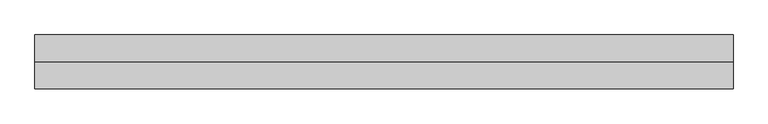
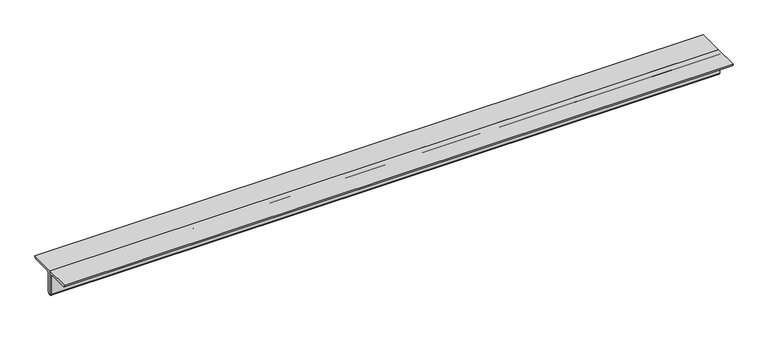
"""IFC4 building model written with IfcOpenShell, lengths in millimetres: member geometry, 0123_Steel Framing_2Ls-KSD3502 : H_SB_AR_S03_2Ls-130x130x12_HBR4."""

from ifc_helpers import new_model, si_unit, point, frame, frame_2d, origin, place, context, project, spatial, polyline, circle_curve, trimmed, segment, composite_curve, outline, extrude, source, transform, mapped, element, save


def member_72eb2c29(model_context):
    return source(origin(), model_context, "Body", "SweptSolid", [
        extrude(outline(composite_curve([segment(polyline([(0.0, 36.4), (130.0, 36.4)]), True, "CONTINUOUS"), segment(trimmed(circle_curve(frame_2d((118.0, 36.4)), 12.0), [point((130.0, 36.4))], [point((118.0, 24.4))], False, "CARTESIAN"), True, "CONTINUOUS"), segment(polyline([(118.0, 24.4), (24.0, 24.4)]), True, "CONTINUOUS"), segment(trimmed(circle_curve(frame_2d((24.0, 12.4)), 12.0), [point((24.0, 24.4))], [point((12.0, 12.4))], True, "CARTESIAN"), True, "CONTINUOUS"), segment(polyline([(12.0, 12.4), (12.0, -81.6)]), True, "CONTINUOUS"), segment(trimmed(circle_curve(frame_2d((0.0, -81.6)), 12.0), [point((12.0, -81.6))], [point((0.0, -93.6))], False, "CARTESIAN"), True, "CONTINUOUS"), segment(polyline([(0.0, -93.6), (0.0, 36.4)]), True, "CONTINUOUS")], self_intersect=False)), frame((-1734.7763172, 0.0, 0.0), z_axis=(1.0, 0.0, 0.0), x_axis=(0.0, 1.0, 0.0)), (0.0, 0.0, 1.0), 3371.9638577),
        extrude(outline(composite_curve([segment(polyline([(0.0, 36.4), (0.0, -93.6)]), True, "CONTINUOUS"), segment(trimmed(circle_curve(frame_2d((0.0, -81.6)), 12.0), [point((0.0, -93.6))], [point((-12.0, -81.6))], False, "CARTESIAN"), True, "CONTINUOUS"), segment(polyline([(-12.0, -81.6), (-12.0, 12.4)]), True, "CONTINUOUS"), segment(trimmed(circle_curve(frame_2d((-24.0, 12.4)), 12.0), [point((-12.0, 12.4))], [point((-24.0, 24.4))], True, "CARTESIAN"), True, "CONTINUOUS"), segment(polyline([(-24.0, 24.4), (-118.0, 24.4)]), True, "CONTINUOUS"), segment(trimmed(circle_curve(frame_2d((-118.0, 36.4)), 12.0), [point((-118.0, 24.4))], [point((-130.0, 36.4))], False, "CARTESIAN"), True, "CONTINUOUS"), segment(polyline([(-130.0, 36.4), (0.0, 36.4)]), True, "CONTINUOUS")], self_intersect=False)), frame((-1734.7763172, 0.0, 0.0), z_axis=(1.0, 0.0, 0.0), x_axis=(0.0, 1.0, 0.0)), (0.0, 0.0, 1.0), 3371.9638577),
    ])


if __name__ == "__main__":
    model = new_model("IFC4")
    model_context = context("Model", 3, world=origin())
    ifc_project = project(units=[si_unit("LENGTHUNIT", "METRE", prefix="MILLI")], contexts=[model_context])
    site = spatial("IfcSite", under=ifc_project)
    building = spatial("IfcBuilding", under=site)
    placement = place(None, origin())
    member_shape = member_72eb2c29(model_context)
    element("IfcMember", 1, ObjectType="0123_Steel Framing_2Ls-KSD3502 : H_SB_AR_S03_2Ls-130x130x12_HBR4", at=placement, inside=building, context=model_context, shape_type="MappedRepresentation", body=[
        mapped(member_shape, transform((0.0, 0.0, 0.0), x_axis=(1.0, 0.0, 0.0), y_axis=(0.0, 1.0, 0.0), z_axis=(0.0, 0.0, 1.0))),
    ])
    save(model, "model.ifc")

# Revit data of these elements
# Type "0123_Steel Framing_2Ls-KSD3502 : H_SB_AR_S03_2Ls-130x130x12_HBR4"
#   Type Mark = "HBR4"
#   Assembly Code = "B10"
#   Legs = "SLBB"
#   W = 8.97
#   Perimeter = 1.04 m²/m
#   Nominal Weight = 46.80 kgf/m
#   Length [instance default] = 1000 mm
#   Space = 0 mm
#   b = 130 mm
#   d = 130 mm
#   t = 12 mm
#   y = 36.4 mm
#   A = 0.005952 m²
#   Structural Material [instance default] = Steel ASTM A36
# Element 1 (IfcMember, "0123_Steel Framing_2Ls-KSD3502 : H_SB_AR_S03_2Ls-130x130x12_HBR4")
#   Materials on its faces: "Steel ASTM A36"
# Materials
#   "Steel ASTM A36": class "Metal", colour RGB 199 199 199, transparency 0, Description = "Structural steel, ASTM A36 Grade B, mill finish", Cost = 0
